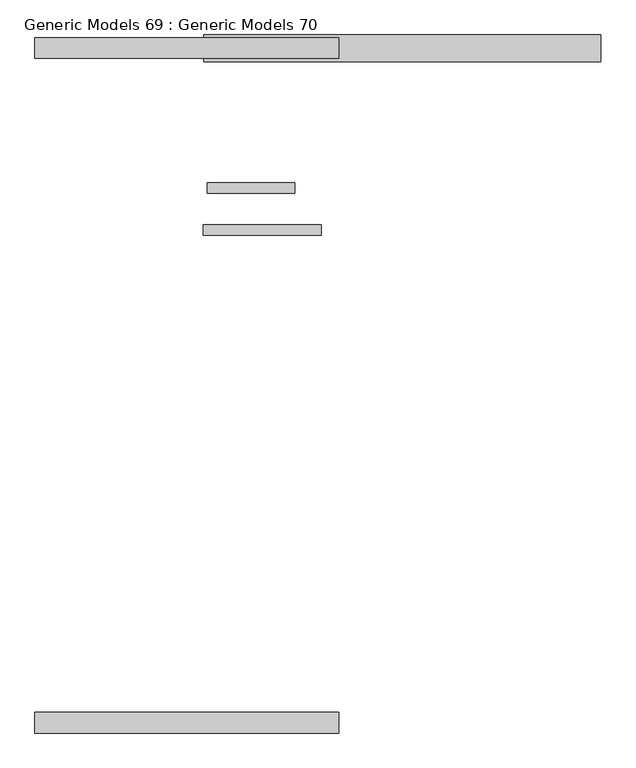
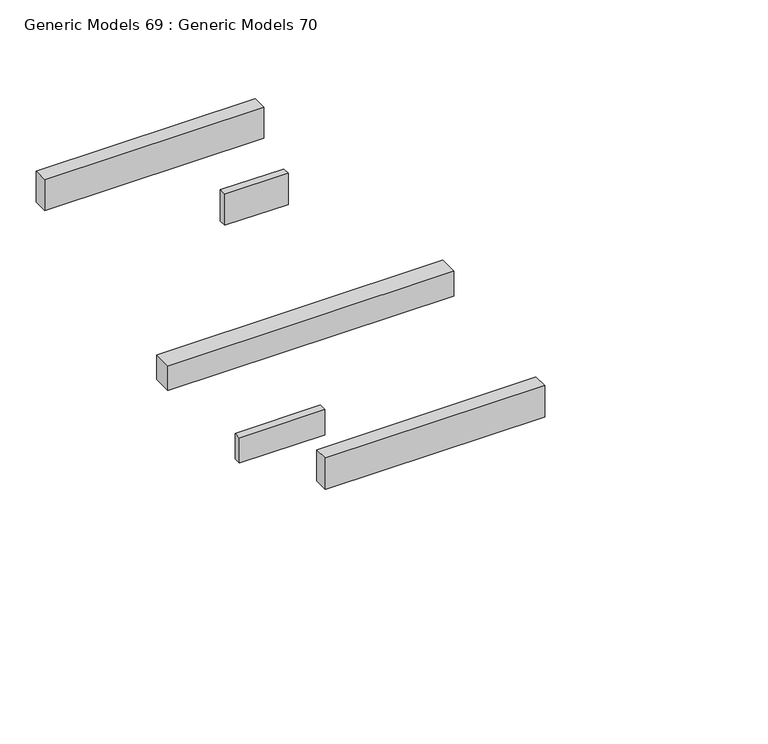
"""IFC4 building model written with IfcOpenShell, lengths in millimetres: proxy geometry, Generic Models 69 : Generic Models 70."""

from ifc_helpers import new_model, si_unit, frame, origin, place, context, project, spatial, polyline, outline, extrude, source, transform, mapped, element, save


def generic_models_69_generic_models_70_647e182c(model_context):
    return source(origin(), model_context, "Body", "SweptSolid", [
        extrude(outline(polyline([(33154.9460525, 34934.2118167), (33154.9460525, 34845.3118167), (32167.5210525, 34845.3118167), (32167.5210525, 34934.2118167), (33154.9460525, 34934.2118167)])), frame((0.0, 0.0, 266065.0), z_axis=(0.0, 0.0, 1.0), x_axis=(1.0, 0.0, 0.0)), (0.0, 0.0, 1.0), 311.15),
        extrude(outline(polyline([(35487.7985365, 36518.5457942), (35487.7985365, 36296.2957942), (32175.4585525, 36296.2957942), (32175.4585525, 36518.5457942), (35487.7985365, 36518.5457942)])), frame((0.0, 0.0, 266071.35), z_axis=(0.0, 0.0, 1.0), x_axis=(1.0, 0.0, 0.0)), (0.0, 0.0, 1.0), 304.8),
        extrude(outline(polyline([(33302.5835525, 36493.1457942), (33302.5835525, 36321.6957942), (30763.3985365, 36321.6957942), (30763.3985365, 36493.1457942), (33302.5835525, 36493.1457942)])), frame((0.0, 0.0, 268757.4), z_axis=(0.0, 0.0, 1.0), x_axis=(1.0, 0.0, 0.0)), (0.0, 0.0, 1.0), 381.0),
        extrude(outline(polyline([(32933.9485589, 35283.4707942), (32933.9485589, 35194.5707942), (32200.8585525, 35194.5707942), (32200.8585525, 35283.4707942), (32933.9485589, 35283.4707942)])), frame((0.0, 0.0, 268757.4), z_axis=(0.0, 0.0, 1.0), x_axis=(1.0, 0.0, 0.0)), (0.0, 0.0, 1.0), 381.0),
        extrude(outline(polyline([(33302.5835525, 30860.0656612), (33302.5835525, 30688.6156612), (30763.3985365, 30688.6156612), (30763.3985365, 30860.0656612), (33302.5835525, 30860.0656612)])), frame((0.0, 0.0, 268757.4), z_axis=(0.0, 0.0, 1.0), x_axis=(1.0, 0.0, 0.0)), (0.0, 0.0, 1.0), 381.0),
    ])


if __name__ == "__main__":
    model = new_model("IFC4")
    model_context = context("Model", 3, world=origin())
    ifc_project = project(units=[si_unit("LENGTHUNIT", "METRE", prefix="MILLI")], contexts=[model_context])
    site = spatial("IfcSite", under=ifc_project)
    building = spatial("IfcBuilding", under=site)
    placement = place(None, origin())
    generic_models_69_generic_models_70_shape = generic_models_69_generic_models_70_647e182c(model_context)
    element("IfcBuildingElementProxy", 1, Name="Generic Models 69 : Generic Models 70", ObjectType="Generic Models 69 : Generic Models 70", at=placement, inside=building, context=model_context, shape_type="MappedRepresentation", body=[
        mapped(generic_models_69_generic_models_70_shape, transform((0.0, 0.0, 0.0), x_axis=(1.0, 0.0, 0.0), y_axis=(0.0, 1.0, 0.0), z_axis=(0.0, 0.0, 1.0))),
    ])
    save(model, "model.ifc")

# Revit data of these elements
# Element 1 (IfcBuildingElementProxy, "Generic Models 69 : Generic Models 70")
#   Materials on its faces: "6 3/4\" x 15\" GLUELAM BEAM", "3 1/2\" x 12\" GLUELAM BEAM", "8 3/4\" x 1' GLUELAM BEAM"
# Materials
#   "6 3/4\" x 15\" GLUELAM BEAM": class "Wood", colour RGB 112 64 44, transparency 0, Description = "Pinus Echinata", Cost = 0
#   "3 1/2\" x 12\" GLUELAM BEAM": class "Wood", colour RGB 214 169 150, transparency 0, Description = "Pinus Echinata", Cost = 0
#   "8 3/4\" x 1' GLUELAM BEAM": class "Wood", colour RGB 112 64 44, transparency 0, Description = "Pinus Echinata", Cost = 0
